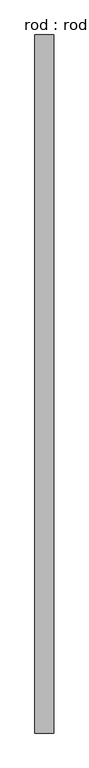
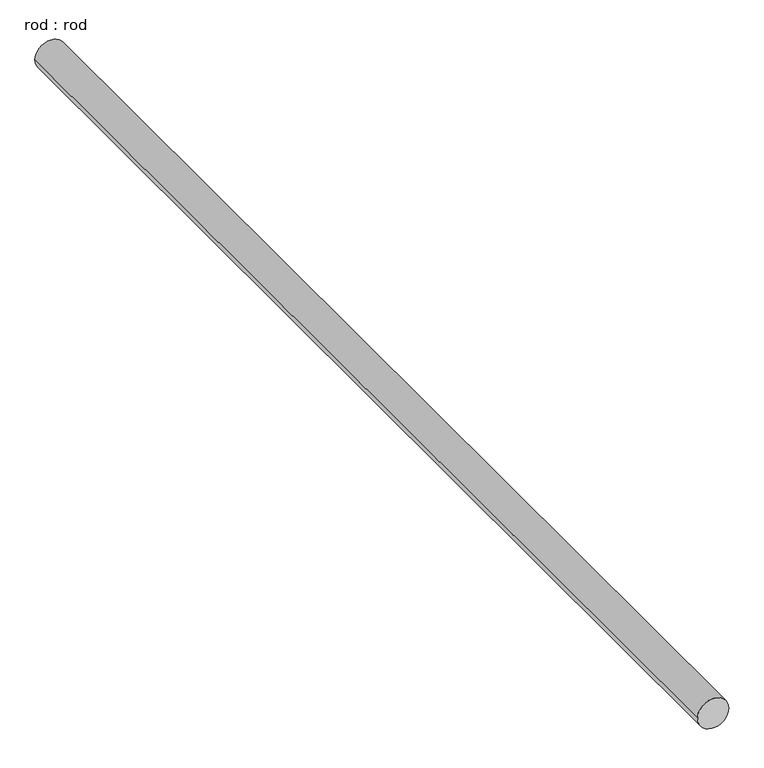
"""IFC4 building model written with IfcOpenShell, lengths in millimetres: proxy geometry, rod : rod."""

from ifc_helpers import new_model, si_unit, point, frame, frame_2d, origin, place, context, project, spatial, circle_curve, trimmed, segment, composite_curve, outline, extrude, source, transform, mapped, element, save


def rod_rod_3e91f297(model_context):
    return source(origin(), model_context, "Body", "SweptSolid", [
        extrude(outline(composite_curve([segment(trimmed(circle_curve(frame_2d((0.0108462, 0.0)), 200.0), [point((0.0108462, 200.0))], [point((0.0108462, -200.0))], False, "CARTESIAN"), True, "CONTINUOUS"), segment(trimmed(circle_curve(frame_2d((0.0108462, 0.0)), 200.0), [point((0.0108462, -200.0))], [point((0.0108462, 200.0))], False, "CARTESIAN"), True, "CONTINUOUS")], self_intersect=False)), frame((0.0, -3278.0451738, 0.0), z_axis=(0.0, 1.0, 0.0), x_axis=(0.0, 0.0, 1.0)), (0.0, 0.0, 1.0), 14741.5475782),
    ])


if __name__ == "__main__":
    model = new_model("IFC4")
    model_context = context("Model", 3, world=origin())
    ifc_project = project(units=[si_unit("LENGTHUNIT", "METRE", prefix="MILLI")], contexts=[model_context])
    site = spatial("IfcSite", under=ifc_project)
    building = spatial("IfcBuilding", under=site)
    placement = place(None, origin())
    rod_rod_shape = rod_rod_3e91f297(model_context)
    element("IfcBuildingElementProxy", 1, Name="rod : rod", ObjectType="rod : rod", at=placement, inside=building, context=model_context, shape_type="MappedRepresentation", body=[
        mapped(rod_rod_shape, transform((0.0, 0.0, 0.0), x_axis=(1.0, 0.0, 0.0), y_axis=(0.0, 1.0, 0.0), z_axis=(0.0, 0.0, 1.0))),
    ])
    save(model, "model.ifc")

# Revit data of these elements
# Type "rod : rod"
#   Default Elevation = 0
